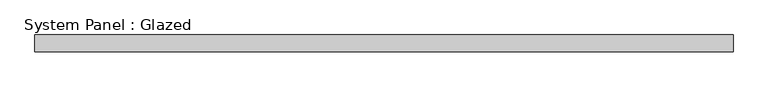
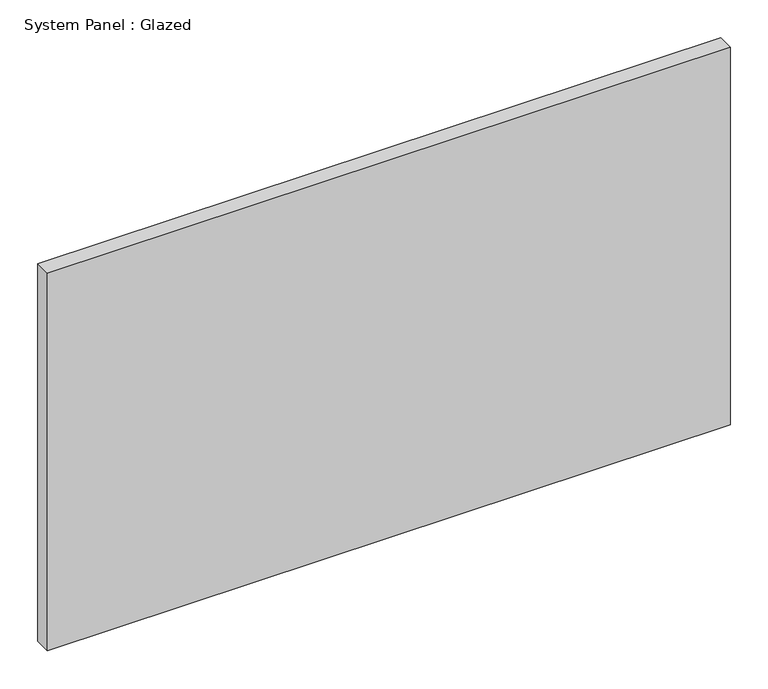
"""IFC4 building model written with IfcOpenShell, lengths in millimetres: plate geometry, System Panel : Glazed."""

import ifcopenshell
import ifcopenshell.guid

model = None  # the IFC model being written
_history = None  # IfcOwnerHistory: only IFC2X3 demands one
_inside = {}  # id of a spatial element -> (the spatial element, [elements in it])
_under = {}  # id of a project, library or spatial element -> (it, [spatial elements below it])
_declared = {}  # id of a project -> (the project, [libraries it declares])
_typed = {}  # id of a type object -> (the type object, [elements of that type])
_made_of = {}  # id of a material, layer set ... -> (it, [elements and type objects made of it])


def new_model(schema):
    """Start an empty IFC model of exactly this schema.

    Asked for "IFC4X3", IfcOpenShell would pick the latest addendum, in which some entities
    have other attributes; the version numbers below select the first issue.
    IFC2X3 requires an IfcOwnerHistory on every rooted entity: one is made here for all.
    """
    global model, _history
    if schema == "IFC4X3":
        model = ifcopenshell.file(schema_version=(4, 3, 0, 0))
    else:
        model = ifcopenshell.file(schema=schema)
    _inside.clear()
    _under.clear()
    _declared.clear()
    _typed.clear()
    _made_of.clear()
    _history = None
    if model.schema == "IFC2X3":
        org = make("IfcOrganization", Name="unknown")
        user = make(
            "IfcPersonAndOrganization",
            ThePerson=make("IfcPerson", FamilyName="unknown"),
            TheOrganization=org,
        )
        app = make(
            "IfcApplication",
            ApplicationDeveloper=org,
            Version="unknown",
            ApplicationFullName="unknown",
            ApplicationIdentifier="unknown",
        )
        _history = make(
            "IfcOwnerHistory",
            OwningUser=user,
            OwningApplication=app,
            ChangeAction="ADDED",
            CreationDate=0,
        )
    return model


def make(cls, **values):
    """One entity of the class cls with the attributes given. An attribute that is None is left unset."""
    return model.create_entity(
        cls, **{name: value for name, value in values.items() if value is not None}
    )


def rooted(cls, **values):
    """An entity with a GlobalId (a new one), such as an element, a storey or a relation."""
    return make(cls, GlobalId=ifcopenshell.guid.new(), OwnerHistory=_history, **values)


def si_unit(unit_type, name, prefix=None):
    """IfcSIUnit, for example si_unit("LENGTHUNIT", "METRE", prefix="MILLI")."""
    return make("IfcSIUnit", UnitType=unit_type, Prefix=prefix, Name=name)


def assignment(units):
    """IfcUnitAssignment: the units of a project."""
    return None if units is None else make("IfcUnitAssignment", Units=units)


def point(xyz):
    """IfcCartesianPoint."""
    return None if xyz is None else make("IfcCartesianPoint", Coordinates=xyz)


def direction(xyz):
    """IfcDirection."""
    return None if xyz is None else make("IfcDirection", DirectionRatios=xyz)


def frame(location, z_axis=None, x_axis=None):
    """IfcAxis2Placement3D, a coordinate frame: its origin and axes. An axis left out is left unset."""
    return make(
        "IfcAxis2Placement3D",
        Location=point(location),
        Axis=direction(z_axis),
        RefDirection=direction(x_axis),
    )


def origin():
    """The frame at (0, 0, 0) with its axes left unset."""
    return frame((0.0, 0.0, 0.0))


def origin_with_axes():
    """The frame at (0, 0, 0) with the z axis (0, 0, 1) and the x axis (1, 0, 0) written out."""
    return frame((0.0, 0.0, 0.0), z_axis=(0.0, 0.0, 1.0), x_axis=(1.0, 0.0, 0.0))


def place(relative_to, where):
    """IfcLocalPlacement: puts the frame where relative to a parent placement (None: the world)."""
    return make(
        "IfcLocalPlacement", PlacementRelTo=relative_to, RelativePlacement=where
    )


def context(
    kind, dimensions, precision=None, world=None, true_north=None, identifier=None
):
    """IfcGeometricRepresentationContext, for example the 3D "Model" context."""
    return make(
        "IfcGeometricRepresentationContext",
        ContextIdentifier=identifier,
        ContextType=kind,
        CoordinateSpaceDimension=dimensions,
        Precision=precision,
        WorldCoordinateSystem=world,
        TrueNorth=true_north,
    )


def project(units=None, contexts=None):
    """IfcProject with its units and contexts."""
    return rooted(
        "IfcProject",
        Name="project",
        RepresentationContexts=contexts,
        UnitsInContext=assignment(units),
    )


def spatial(cls, under=None, at=None, **own):
    """A site, building, storey or space (cls), placed at a placement, below another one or the project."""
    s = rooted(cls, ObjectPlacement=at, **own)
    if under is not None:
        _under.setdefault(under.id(), (under, []))[1].append(s)
    return s


def polyline(points):
    """IfcPolyline through the points."""
    return make("IfcPolyline", Points=[point(p) for p in points])


def outline(outer, holes=None, kind="AREA"):
    """IfcArbitraryClosedProfileDef: a profile drawn as a closed curve; with holes, ...WithVoids."""
    if holes is None:
        return make("IfcArbitraryClosedProfileDef", ProfileType=kind, OuterCurve=outer)
    return make(
        "IfcArbitraryProfileDefWithVoids",
        ProfileType=kind,
        OuterCurve=outer,
        InnerCurves=holes,
    )


def extrude(swept, where, along, depth):
    """IfcExtrudedAreaSolid: the profile swept, set in the frame where, extruded along a direction by depth."""
    return make(
        "IfcExtrudedAreaSolid",
        SweptArea=swept,
        Position=where,
        ExtrudedDirection=direction(along),
        Depth=depth,
    )


def shape(context_of_items, identifier, shape_type, items):
    """IfcShapeRepresentation: the items that make up one representation, for example the "Body"."""
    return make(
        "IfcShapeRepresentation",
        ContextOfItems=context_of_items,
        RepresentationIdentifier=identifier,
        RepresentationType=shape_type,
        Items=items,
    )


def source(mapping_origin, context_of_items, identifier, shape_type, items):
    """IfcRepresentationMap: a shape defined once, which mapped items show again and again."""
    return make(
        "IfcRepresentationMap",
        MappingOrigin=mapping_origin,
        MappedRepresentation=shape(context_of_items, identifier, shape_type, items),
    )


def transform(
    local_origin,
    x_axis=None,
    y_axis=None,
    z_axis=None,
    scale=None,
    scale2=None,
    scale3=None,
    uniform=True,
):
    """IfcCartesianTransformationOperator3D, or its non-uniform kind. x_axis, y_axis, z_axis: its Axis1, 2, 3."""
    if uniform:
        return make(
            "IfcCartesianTransformationOperator3D",
            Axis1=direction(x_axis),
            Axis2=direction(y_axis),
            LocalOrigin=point(local_origin),
            Scale=scale,
            Axis3=direction(z_axis),
        )
    return make(
        "IfcCartesianTransformationOperator3DnonUniform",
        Axis1=direction(x_axis),
        Axis2=direction(y_axis),
        LocalOrigin=point(local_origin),
        Scale=scale,
        Axis3=direction(z_axis),
        Scale2=scale2,
        Scale3=scale3,
    )


def mapped(mapping_source, mapping_target):
    """IfcMappedItem: shows the shape of a source again, moved by a transform."""
    return make(
        "IfcMappedItem", MappingSource=mapping_source, MappingTarget=mapping_target
    )


def made_of(thing, what):
    """Note that an element or type object is made of a material, layer set ...; save() writes the relation."""
    if what is not None:
        _made_of.setdefault(what.id(), (what, []))[1].append(thing)
    return thing


def element(
    cls,
    number,
    at=None,
    inside=None,
    cuts=None,
    type_object=None,
    material=None,
    context=None,
    identifier="Body",
    shape_type=None,
    held_by="IfcProductDefinitionShape",
    body=None,
    shapes=None,
    **own,
):
    """One element of the class cls, such as IfcWall. Its Tag is "e" and its number.

    at: its placement. inside: the storey or other place that contains it. cuts: it is an
    opening in that element (IfcRelVoidsElement). A single representation is given by context,
    identifier, shape_type and body (its items); several are given by shapes. held_by: the class
    of the entity that holds the representations. save() writes the other relations.
    """
    e = rooted(cls, Tag="e%d" % number, ObjectPlacement=at, **own)
    if body is not None:
        shapes = [shape(context, identifier, shape_type, body)]
    if shapes is not None:
        e.Representation = make(held_by, Representations=shapes)
    if inside is not None:
        _inside.setdefault(inside.id(), (inside, []))[1].append(e)
    if cuts is not None:
        rooted(
            "IfcRelVoidsElement", RelatingBuildingElement=cuts, RelatedOpeningElement=e
        )
    if type_object is not None:
        _typed.setdefault(type_object.id(), (type_object, []))[1].append(e)
    return made_of(e, material)


def aggregate(whole, parts):
    """IfcRelAggregates: a whole, such as a stair, and the parts it consists of."""
    return rooted("IfcRelAggregates", RelatingObject=whole, RelatedObjects=parts)


def save(model, path):
    """Write the relations noted so far, then the file.

    IfcRelAggregates (storeys below a building ...), IfcRelContainedInSpatialStructure (elements
    in a storey), IfcRelDefinesByType, IfcRelAssociatesMaterial and IfcRelDeclares: one each for
    every whole, place, type object, material and project.
    """
    for whole, parts in _under.values():
        aggregate(whole, parts)
    for where, things in _inside.values():
        rooted(
            "IfcRelContainedInSpatialStructure",
            RelatedElements=things,
            RelatingStructure=where,
        )
    for kind, things in _typed.values():
        rooted("IfcRelDefinesByType", RelatedObjects=things, RelatingType=kind)
    for what, things in _made_of.values():
        rooted("IfcRelAssociatesMaterial", RelatedObjects=things, RelatingMaterial=what)
    for by, libraries in _declared.values():
        rooted("IfcRelDeclares", RelatingContext=by, RelatedDefinitions=libraries)
    model.write(path)


def system_panel_glazed_8af3892a(model_context):
    return source(origin(), model_context, "Body", "SweptSolid", [
        extrude(outline(polyline([(521.5143964, 19.05), (-521.5143964, 19.05), (-521.5143964, 44.45), (521.5143964, 44.45), (521.5143964, 19.05)])), origin_with_axes(), (0.0, 0.0, 1.0), 609.6),
    ])


if __name__ == "__main__":
    model = new_model("IFC4")
    model_context = context("Model", 3, world=origin())
    ifc_project = project(units=[si_unit("LENGTHUNIT", "METRE", prefix="MILLI")], contexts=[model_context])
    site = spatial("IfcSite", under=ifc_project)
    building = spatial("IfcBuilding", under=site)
    placement = place(None, origin())
    system_panel_glazed_shape = system_panel_glazed_8af3892a(model_context)
    element("IfcPlate", 1, ObjectType="System Panel : Glazed", at=placement, inside=building, context=model_context, shape_type="MappedRepresentation", body=[
        mapped(system_panel_glazed_shape, transform((0.0, 0.0, 0.0), x_axis=(1.0, 0.0, 0.0), y_axis=(0.0, 1.0, 0.0), z_axis=(0.0, 0.0, 1.0))),
    ])
    save(model, "model.ifc")

# Revit data of these elements
# Element 1 (IfcPlate, "System Panel : Glazed")
#   Materials on its faces: "Glass"
# Materials
#   "Glass": class "Glass", colour RGB 0 128 192, transparency 0.75
